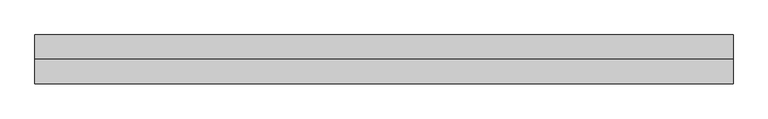
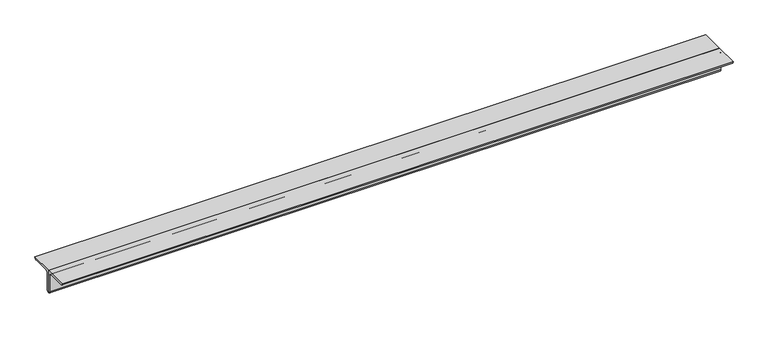
"""IFC4 building model written with IfcOpenShell, lengths in millimetres: member geometry, 0123_Steel Framing_2Ls-KSD3502 : H_SB_AR_S03_2Ls-130x130x12_HBR1."""

from ifc_helpers import new_model, si_unit, point, frame, frame_2d, origin, place, context, project, spatial, polyline, circle_curve, trimmed, segment, composite_curve, outline, extrude, source, transform, mapped, element, save


def member_2dd2a1f8(model_context):
    return source(origin(), model_context, "Body", "SweptSolid", [
        extrude(outline(composite_curve([segment(polyline([(0.0, 36.4), (0.0, -93.6)]), True, "CONTINUOUS"), segment(trimmed(circle_curve(frame_2d((0.0, -81.6)), 12.0), [point((0.0, -93.6))], [point((-12.0, -81.6))], False, "CARTESIAN"), True, "CONTINUOUS"), segment(polyline([(-12.0, -81.6), (-12.0, 12.4)]), True, "CONTINUOUS"), segment(trimmed(circle_curve(frame_2d((-24.0, 12.4)), 12.0), [point((-12.0, 12.4))], [point((-24.0, 24.4))], True, "CARTESIAN"), True, "CONTINUOUS"), segment(polyline([(-24.0, 24.4), (-118.0, 24.4)]), True, "CONTINUOUS"), segment(trimmed(circle_curve(frame_2d((-118.0, 36.4)), 12.0), [point((-118.0, 24.4))], [point((-130.0, 36.4))], False, "CARTESIAN"), True, "CONTINUOUS"), segment(polyline([(-130.0, 36.4), (0.0, 36.4)]), True, "CONTINUOUS")], self_intersect=False)), frame((-1830.7666695, 0.0, 0.0), z_axis=(1.0, 0.0, 0.0), x_axis=(0.0, 1.0, 0.0)), (0.0, 0.0, 1.0), 3701.6272171),
        extrude(outline(composite_curve([segment(polyline([(0.0, 36.4), (130.0, 36.4)]), True, "CONTINUOUS"), segment(trimmed(circle_curve(frame_2d((118.0, 36.4)), 12.0), [point((130.0, 36.4))], [point((118.0, 24.4))], False, "CARTESIAN"), True, "CONTINUOUS"), segment(polyline([(118.0, 24.4), (24.0, 24.4)]), True, "CONTINUOUS"), segment(trimmed(circle_curve(frame_2d((24.0, 12.4)), 12.0), [point((24.0, 24.4))], [point((12.0, 12.4))], True, "CARTESIAN"), True, "CONTINUOUS"), segment(polyline([(12.0, 12.4), (12.0, -81.6)]), True, "CONTINUOUS"), segment(trimmed(circle_curve(frame_2d((0.0, -81.6)), 12.0), [point((12.0, -81.6))], [point((0.0, -93.6))], False, "CARTESIAN"), True, "CONTINUOUS"), segment(polyline([(0.0, -93.6), (0.0, 36.4)]), True, "CONTINUOUS")], self_intersect=False)), frame((-1830.7666695, 0.0, 0.0), z_axis=(1.0, 0.0, 0.0), x_axis=(0.0, 1.0, 0.0)), (0.0, 0.0, 1.0), 3701.6272171),
    ])


if __name__ == "__main__":
    model = new_model("IFC4")
    model_context = context("Model", 3, world=origin())
    ifc_project = project(units=[si_unit("LENGTHUNIT", "METRE", prefix="MILLI")], contexts=[model_context])
    site = spatial("IfcSite", under=ifc_project)
    building = spatial("IfcBuilding", under=site)
    placement = place(None, origin())
    member_shape = member_2dd2a1f8(model_context)
    element("IfcMember", 1, ObjectType="0123_Steel Framing_2Ls-KSD3502 : H_SB_AR_S03_2Ls-130x130x12_HBR1", at=placement, inside=building, context=model_context, shape_type="MappedRepresentation", body=[
        mapped(member_shape, transform((0.0, 0.0, 0.0), x_axis=(1.0, 0.0, 0.0), y_axis=(0.0, 1.0, 0.0), z_axis=(0.0, 0.0, 1.0))),
    ])
    save(model, "model.ifc")

# Revit data of these elements
# Type "0123_Steel Framing_2Ls-KSD3502 : H_SB_AR_S03_2Ls-130x130x12_HBR1"
#   Type Mark = "HBR1"
#   Assembly Code = "B10"
#   Legs = "SLBB"
#   W = 8.97
#   Perimeter = 1.04 m²/m
#   Nominal Weight = 46.80 kgf/m
#   Length [instance default] = 1000 mm
#   Space = 0 mm
#   b = 130 mm
#   d = 130 mm
#   t = 12 mm
#   y = 36.4 mm
#   A = 0.005952 m²
#   Structural Material [instance default] = Steel ASTM A36
# Element 1 (IfcMember, "0123_Steel Framing_2Ls-KSD3502 : H_SB_AR_S03_2Ls-130x130x12_HBR1")
#   Materials on its faces: "Steel ASTM A36"
# Materials
#   "Steel ASTM A36": class "Metal", colour RGB 199 199 199, transparency 0, Description = "Structural steel, ASTM A36 Grade B, mill finish", Cost = 0
